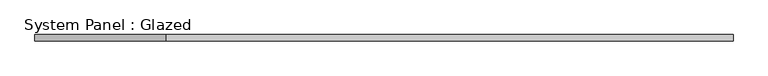
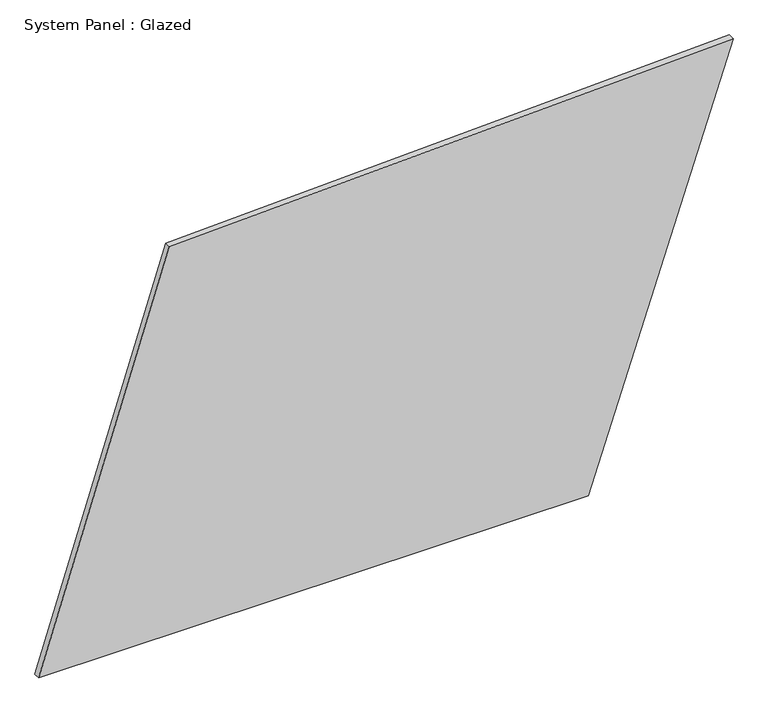
"""IFC4 building model written with IfcOpenShell, lengths in millimetres: plate geometry, System Panel : Glazed."""

from ifc_helpers import new_model, si_unit, frame, origin, place, context, project, spatial, polyline, outline, extrude, source, transform, mapped, element, save


def system_panel_glazed_05480fd8(model_context):
    return source(origin(), model_context, "Body", "SweptSolid", [
        extrude(outline(polyline([(0.0, -1345.9129878), (0.0, 784.5031912), (1677.5728739, 1345.9129878), (1589.6338357, -839.6823282), (0.0, -1345.9129878)])), frame((0.0, -49.5, 0.0), z_axis=(0.0, 1.0, 0.0), x_axis=(0.0, 0.0, 1.0)), (0.0, 0.0, 1.0), 25.0),
    ])


if __name__ == "__main__":
    model = new_model("IFC4")
    model_context = context("Model", 3, world=origin())
    ifc_project = project(units=[si_unit("LENGTHUNIT", "METRE", prefix="MILLI")], contexts=[model_context])
    site = spatial("IfcSite", under=ifc_project)
    building = spatial("IfcBuilding", under=site)
    placement = place(None, origin())
    system_panel_glazed_shape = system_panel_glazed_05480fd8(model_context)
    element("IfcPlate", 1, ObjectType="System Panel : Glazed", at=placement, inside=building, context=model_context, shape_type="MappedRepresentation", body=[
        mapped(system_panel_glazed_shape, transform((0.0, 0.0, 0.0), x_axis=(1.0, 0.0, 0.0), y_axis=(0.0, 1.0, 0.0), z_axis=(0.0, 0.0, 1.0))),
    ])
    save(model, "model.ifc")

# Revit data of these elements
# Element 1 (IfcPlate, "System Panel : Glazed")
#   Materials on its faces: "Glass, Clear Glazing"
# Materials
#   "Glass, Clear Glazing": class "Glass", colour RGB 247 249 248, transparency 0.85, Description = "Clear glazing", Cost = 0
